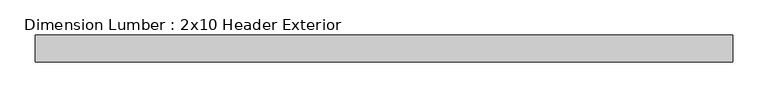
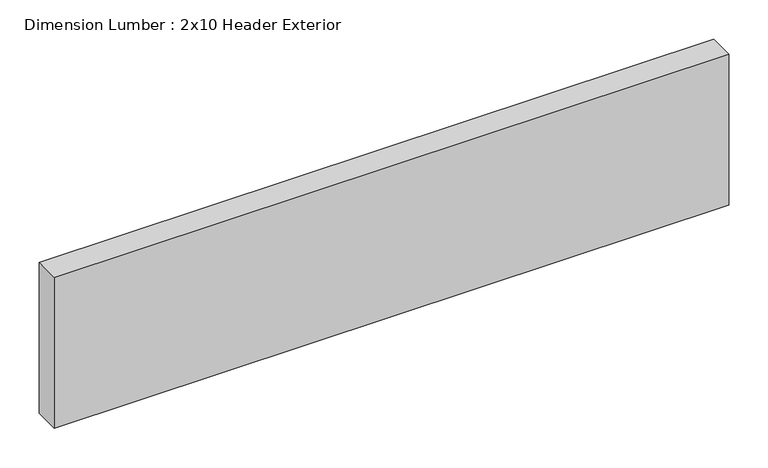
"""IFC4 building model written with IfcOpenShell, lengths in millimetres: beam geometry, Dimension Lumber : 2x10 Header Exterior."""

from ifc_helpers import new_model, si_unit, frame, origin, place, context, project, spatial, polyline, outline, extrude, source, transform, mapped, element, save


def dimension_lumber_2x10_header_exterior_3e47137c(model_context):
    return source(origin(), model_context, "Body", "SweptSolid", [
        extrude(outline(polyline([(468.709375, 19.05), (468.709375, -19.05), (-521.890625, -19.05), (-521.890625, 19.05), (468.709375, 19.05)])), frame((0.0, 0.0, -117.475), z_axis=(0.0, 0.0, 1.0), x_axis=(1.0, 0.0, 0.0)), (0.0, 0.0, 1.0), 234.95),
    ])


if __name__ == "__main__":
    model = new_model("IFC4")
    model_context = context("Model", 3, world=origin())
    ifc_project = project(units=[si_unit("LENGTHUNIT", "METRE", prefix="MILLI")], contexts=[model_context])
    site = spatial("IfcSite", under=ifc_project)
    building = spatial("IfcBuilding", under=site)
    placement = place(None, origin())
    dimension_lumber_2x10_header_exterior_shape = dimension_lumber_2x10_header_exterior_3e47137c(model_context)
    element("IfcBeam", 1, ObjectType="Dimension Lumber : 2x10 Header Exterior", at=placement, inside=building, context=model_context, shape_type="MappedRepresentation", body=[
        mapped(dimension_lumber_2x10_header_exterior_shape, transform((0.0, 0.0, 0.0), x_axis=(1.0, 0.0, 0.0), y_axis=(0.0, 1.0, 0.0), z_axis=(0.0, 0.0, 1.0))),
    ])
    save(model, "model.ifc")

# Revit data of these elements
# Type "Dimension Lumber : 2x10 Header Exterior"
#   Assembly Code = "B10"
#   A = 0.0963889 SF
#   Length [instance default] = 5' - 0"
#   b = 0' - 1 1/2"
#   d = 0' - 9 1/4"
#   Structural Material [instance default] = Softwood, Lumber
# Element 1 (IfcBeam, "Dimension Lumber : 2x10 Header Exterior")
#   Structural Material = Douglas Fir #2
#   Materials on its faces: "Douglas Fir #2"
# Materials
#   "Softwood, Lumber": class "Wood", colour RGB 223 192 134, transparency 0, Description = "Pinus Echinata", Cost = 0
#   "Douglas Fir #2": class "Wood", colour RGB 223 192 134, transparency 0, Description = "Pinus Echinata", Cost = 0
